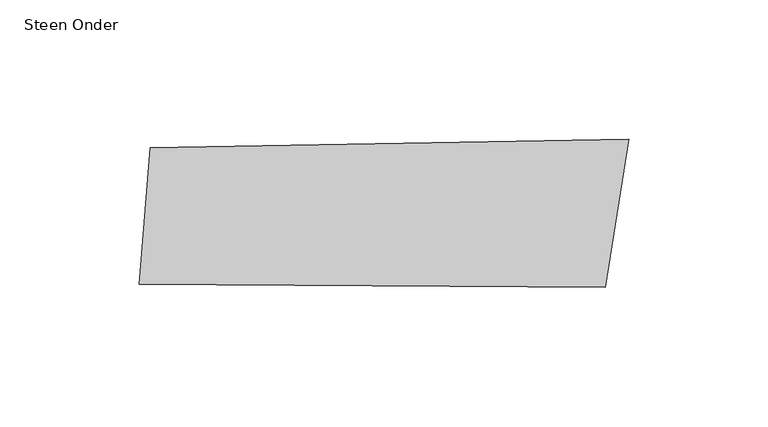
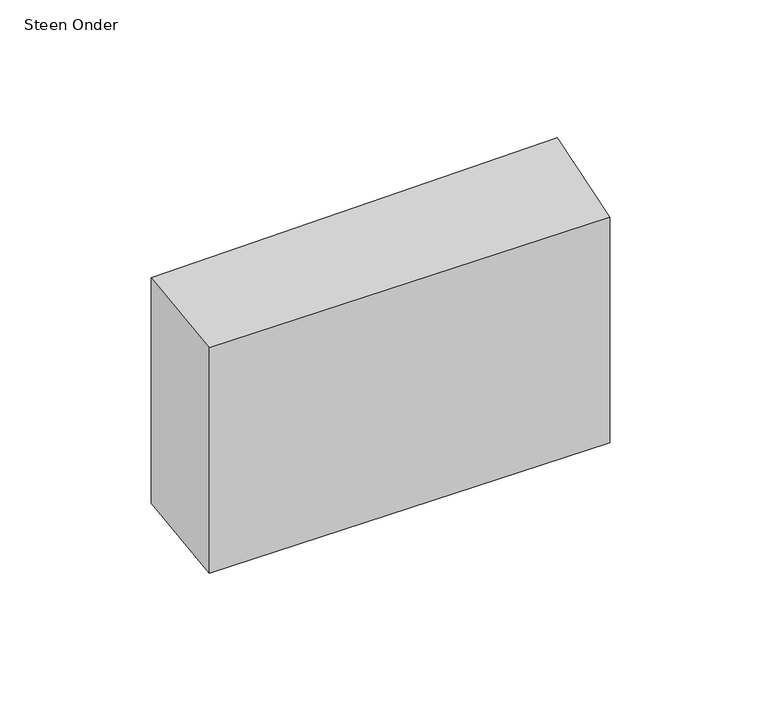
"""IFC4 building model written with IfcOpenShell, lengths in millimetres: proxy geometry, 00_GMA_steen_versie_4 : Steen Onder."""

from ifc_helpers import new_model, si_unit, frame, origin, place, context, project, spatial, polyline, outline, extrude, source, transform, mapped, element, save


def steen_onder_f86a6818(model_context):
    return source(origin(), model_context, "Body", "SweptSolid", [
        extrude(outline(polyline([(188.5451899, 65.0866895), (180.007754, 11.8820728), (12.6551521, 12.9464116), (16.6239761, 62.0803648), (188.5451899, 65.0866895)])), frame((0.0, 0.0, -100.0), z_axis=(0.0, 0.0, 1.0), x_axis=(1.0, 0.0, 0.0)), (0.0, 0.0, 1.0), 100.0),
    ])


if __name__ == "__main__":
    model = new_model("IFC4")
    model_context = context("Model", 3, world=origin())
    ifc_project = project(units=[si_unit("LENGTHUNIT", "METRE", prefix="MILLI")], contexts=[model_context])
    site = spatial("IfcSite", under=ifc_project)
    building = spatial("IfcBuilding", under=site)
    placement = place(None, origin())
    steen_onder_shape = steen_onder_f86a6818(model_context)
    element("IfcBuildingElementProxy", 1, Name="00_GMA_steen_versie_4 : Steen Onder", ObjectType="00_GMA_steen_versie_4 : Steen Onder", at=placement, inside=building, context=model_context, shape_type="MappedRepresentation", body=[
        mapped(steen_onder_shape, transform((0.0, 0.0, 0.0), x_axis=(1.0, 0.0, 0.0), y_axis=(0.0, 1.0, 0.0), z_axis=(0.0, 0.0, 1.0))),
    ])
    save(model, "model.ifc")

# Revit data of these elements
# Type "00_GMA_steen_versie_4 : Steen Onder"
#   StootVoegHalfBoven [instance default] = 5 mm
#   StootVoegHalf [instance default] = 5 mm
#   StootVoegBreedteOnder = 10 mm
#   StootVoegBreedteBoven = 10 mm
#   Steendikte = 100 mm
#   LintVoegOnderHalf = 0 mm
#   LintVoegOnder = 0 mm
#   LintVoegBovenHalf = 5 mm
#   LintVoegBoven = 10 mm
#   materiaal = none
#   MateriaalVoeg = none
#   Default Elevation = 0
